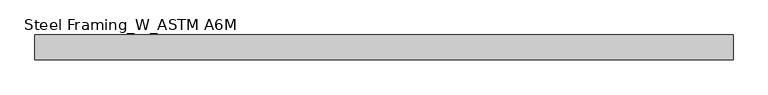
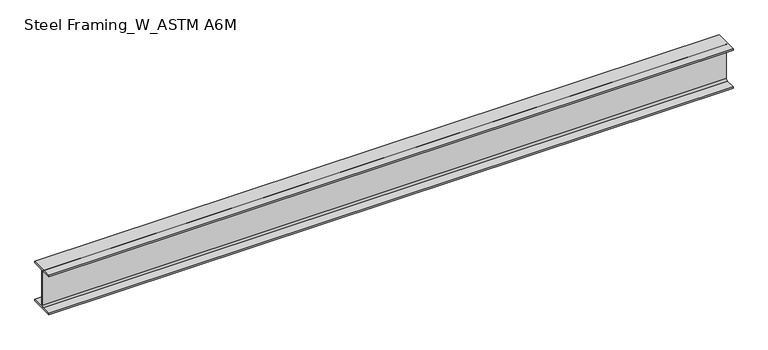
"""IFC4 building model written with IfcOpenShell, lengths in millimetres: beam geometry, Steel Framing_W_ASTM A6M : H_SB_ASB_W360x64."""

from ifc_helpers import new_model, si_unit, point, frame, frame_2d, origin, place, context, project, spatial, polyline, circle_curve, trimmed, segment, composite_curve, outline, extrude, source, transform, mapped, element, save


def steel_framing_w_astm_a6m_73cd2dcb(model_context):
    return source(origin(), model_context, "Body", "SweptSolid", [
        extrude(outline(composite_curve([segment(polyline([(101.5, -160.5), (101.5, -174.0), (-101.5, -174.0), (-101.5, -160.5), (-18.775, -160.5)]), True, "CONTINUOUS"), segment(trimmed(circle_curve(frame_2d((-18.775, -145.6)), 14.9), [point((-18.775, -160.5))], [point((-3.875, -145.6))], True, "CARTESIAN"), True, "CONTINUOUS"), segment(polyline([(-3.875, -145.6), (-3.875, 145.6)]), True, "CONTINUOUS"), segment(trimmed(circle_curve(frame_2d((-18.775, 145.6)), 14.9), [point((-3.875, 145.6))], [point((-18.775, 160.5))], True, "CARTESIAN"), True, "CONTINUOUS"), segment(polyline([(-18.775, 160.5), (-101.5, 160.5), (-101.5, 174.0), (101.5, 174.0), (101.5, 160.5), (18.775, 160.5)]), True, "CONTINUOUS"), segment(trimmed(circle_curve(frame_2d((18.775, 145.6)), 14.9), [point((18.775, 160.5))], [point((3.875, 145.6))], True, "CARTESIAN"), True, "CONTINUOUS"), segment(polyline([(3.875, 145.6), (3.875, -145.6)]), True, "CONTINUOUS"), segment(trimmed(circle_curve(frame_2d((18.775, -145.6)), 14.9), [point((3.875, -145.6))], [point((18.775, -160.5))], True, "CARTESIAN"), True, "CONTINUOUS"), segment(polyline([(18.775, -160.5), (101.5, -160.5)]), True, "CONTINUOUS")], self_intersect=False)), frame((-2795.05, 0.0, 0.0), z_axis=(1.0, 0.0, 0.0), x_axis=(0.0, 1.0, 0.0)), (0.0, 0.0, 1.0), 5695.2),
    ])


if __name__ == "__main__":
    model = new_model("IFC4")
    model_context = context("Model", 3, world=origin())
    ifc_project = project(units=[si_unit("LENGTHUNIT", "METRE", prefix="MILLI")], contexts=[model_context])
    site = spatial("IfcSite", under=ifc_project)
    building = spatial("IfcBuilding", under=site)
    placement = place(None, origin())
    steel_framing_w_astm_a6m_shape = steel_framing_w_astm_a6m_73cd2dcb(model_context)
    element("IfcBeam", 1, ObjectType="Steel Framing_W_ASTM A6M : H_SB_ASB_W360x64", at=placement, inside=building, context=model_context, shape_type="MappedRepresentation", body=[
        mapped(steel_framing_w_astm_a6m_shape, transform((0.0, 0.0, 0.0), x_axis=(1.0, 0.0, 0.0), y_axis=(0.0, 1.0, 0.0), z_axis=(0.0, 0.0, 1.0))),
    ])
    save(model, "model.ifc")

# Revit data of these elements
# Type "Steel Framing_W_ASTM A6M : H_SB_ASB_W360x64"
#   Section Name Key = "W14x43"
#   Width = 20.3 cm
#   Web Thickness = 0.775 cm
#   Web Fillet = 1.49 cm
#   Warping Constant = 524000.0 cm⁶
#   Torsional Moment of Inertia = 43.70 cm⁴
#   Section Area = 81.3 cm²
#   Plastic Modulus weak axis = 283.0 cm³
#   Plastic Modulus strong axis = 1140.0 cm³
#   Perimeter = 1.47 m²/m
#   Nominal Weight = 64.00 kgf/m
#   Moment of Inertia weak axis = 1880.00 cm⁴
#   Moment of Inertia strong axis = 17800.00 cm⁴
#   Height = 34.8 cm
#   Flange Thickness = 1.35 cm
#   Elastic Modulus weak axis = 185.0 cm³
#   Elastic Modulus strong axis = 1030.0 cm³
#   Centroid Vertical = 17.4 cm
#   Centroid Horizontal = 10.15 cm
#   Length [instance default] = 1500.000 mm
#   Structural Material [instance default] = Steel, 45-345
#   Bolt Spacing = 0
#   Assembly Code = ""
# Element 1 (IfcBeam, "Steel Framing_W_ASTM A6M : H_SB_ASB_W360x64")
#   Materials on its faces: "Steel, 45-345"
# Materials
#   "Steel, 45-345": class "Metal", colour RGB 189 187 185, transparency 0, Description = "Steel 345 MPa", Cost = 0
